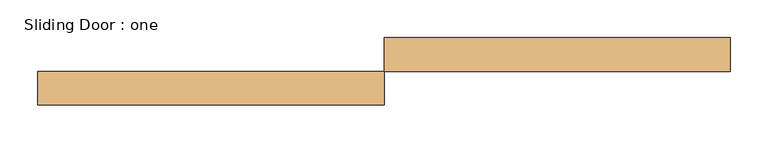
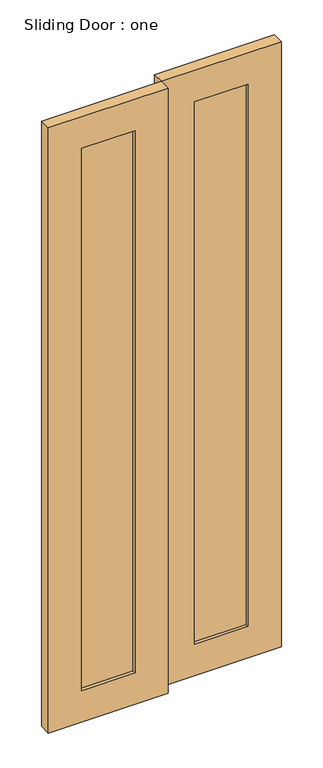
"""IFC4 building model written with IfcOpenShell, lengths in millimetres: door geometry, Sliding Door : one."""

import ifcopenshell
import ifcopenshell.guid

model = None  # the IFC model being written
_history = None  # IfcOwnerHistory: only IFC2X3 demands one
_inside = {}  # id of a spatial element -> (the spatial element, [elements in it])
_under = {}  # id of a project, library or spatial element -> (it, [spatial elements below it])
_declared = {}  # id of a project -> (the project, [libraries it declares])
_typed = {}  # id of a type object -> (the type object, [elements of that type])
_made_of = {}  # id of a material, layer set ... -> (it, [elements and type objects made of it])


def new_model(schema):
    """Start an empty IFC model of exactly this schema.

    Asked for "IFC4X3", IfcOpenShell would pick the latest addendum, in which some entities
    have other attributes; the version numbers below select the first issue.
    IFC2X3 requires an IfcOwnerHistory on every rooted entity: one is made here for all.
    """
    global model, _history
    if schema == "IFC4X3":
        model = ifcopenshell.file(schema_version=(4, 3, 0, 0))
    else:
        model = ifcopenshell.file(schema=schema)
    _inside.clear()
    _under.clear()
    _declared.clear()
    _typed.clear()
    _made_of.clear()
    _history = None
    if model.schema == "IFC2X3":
        org = make("IfcOrganization", Name="unknown")
        user = make(
            "IfcPersonAndOrganization",
            ThePerson=make("IfcPerson", FamilyName="unknown"),
            TheOrganization=org,
        )
        app = make(
            "IfcApplication",
            ApplicationDeveloper=org,
            Version="unknown",
            ApplicationFullName="unknown",
            ApplicationIdentifier="unknown",
        )
        _history = make(
            "IfcOwnerHistory",
            OwningUser=user,
            OwningApplication=app,
            ChangeAction="ADDED",
            CreationDate=0,
        )
    return model


def make(cls, **values):
    """One entity of the class cls with the attributes given. An attribute that is None is left unset."""
    return model.create_entity(
        cls, **{name: value for name, value in values.items() if value is not None}
    )


def rooted(cls, **values):
    """An entity with a GlobalId (a new one), such as an element, a storey or a relation."""
    return make(cls, GlobalId=ifcopenshell.guid.new(), OwnerHistory=_history, **values)


def si_unit(unit_type, name, prefix=None):
    """IfcSIUnit, for example si_unit("LENGTHUNIT", "METRE", prefix="MILLI")."""
    return make("IfcSIUnit", UnitType=unit_type, Prefix=prefix, Name=name)


def assignment(units):
    """IfcUnitAssignment: the units of a project."""
    return None if units is None else make("IfcUnitAssignment", Units=units)


def point(xyz):
    """IfcCartesianPoint."""
    return None if xyz is None else make("IfcCartesianPoint", Coordinates=xyz)


def direction(xyz):
    """IfcDirection."""
    return None if xyz is None else make("IfcDirection", DirectionRatios=xyz)


def frame(location, z_axis=None, x_axis=None):
    """IfcAxis2Placement3D, a coordinate frame: its origin and axes. An axis left out is left unset."""
    return make(
        "IfcAxis2Placement3D",
        Location=point(location),
        Axis=direction(z_axis),
        RefDirection=direction(x_axis),
    )


def origin():
    """The frame at (0, 0, 0) with its axes left unset."""
    return frame((0.0, 0.0, 0.0))


def place(relative_to, where):
    """IfcLocalPlacement: puts the frame where relative to a parent placement (None: the world)."""
    return make(
        "IfcLocalPlacement", PlacementRelTo=relative_to, RelativePlacement=where
    )


def context(
    kind, dimensions, precision=None, world=None, true_north=None, identifier=None
):
    """IfcGeometricRepresentationContext, for example the 3D "Model" context."""
    return make(
        "IfcGeometricRepresentationContext",
        ContextIdentifier=identifier,
        ContextType=kind,
        CoordinateSpaceDimension=dimensions,
        Precision=precision,
        WorldCoordinateSystem=world,
        TrueNorth=true_north,
    )


def project(units=None, contexts=None):
    """IfcProject with its units and contexts."""
    return rooted(
        "IfcProject",
        Name="project",
        RepresentationContexts=contexts,
        UnitsInContext=assignment(units),
    )


def spatial(cls, under=None, at=None, **own):
    """A site, building, storey or space (cls), placed at a placement, below another one or the project."""
    s = rooted(cls, ObjectPlacement=at, **own)
    if under is not None:
        _under.setdefault(under.id(), (under, []))[1].append(s)
    return s


def polyline(points):
    """IfcPolyline through the points."""
    return make("IfcPolyline", Points=[point(p) for p in points])


def outline(outer, holes=None, kind="AREA"):
    """IfcArbitraryClosedProfileDef: a profile drawn as a closed curve; with holes, ...WithVoids."""
    if holes is None:
        return make("IfcArbitraryClosedProfileDef", ProfileType=kind, OuterCurve=outer)
    return make(
        "IfcArbitraryProfileDefWithVoids",
        ProfileType=kind,
        OuterCurve=outer,
        InnerCurves=holes,
    )


def extrude(swept, where, along, depth):
    """IfcExtrudedAreaSolid: the profile swept, set in the frame where, extruded along a direction by depth."""
    return make(
        "IfcExtrudedAreaSolid",
        SweptArea=swept,
        Position=where,
        ExtrudedDirection=direction(along),
        Depth=depth,
    )


def shape(context_of_items, identifier, shape_type, items):
    """IfcShapeRepresentation: the items that make up one representation, for example the "Body"."""
    return make(
        "IfcShapeRepresentation",
        ContextOfItems=context_of_items,
        RepresentationIdentifier=identifier,
        RepresentationType=shape_type,
        Items=items,
    )


def source(mapping_origin, context_of_items, identifier, shape_type, items):
    """IfcRepresentationMap: a shape defined once, which mapped items show again and again."""
    return make(
        "IfcRepresentationMap",
        MappingOrigin=mapping_origin,
        MappedRepresentation=shape(context_of_items, identifier, shape_type, items),
    )


def transform(
    local_origin,
    x_axis=None,
    y_axis=None,
    z_axis=None,
    scale=None,
    scale2=None,
    scale3=None,
    uniform=True,
):
    """IfcCartesianTransformationOperator3D, or its non-uniform kind. x_axis, y_axis, z_axis: its Axis1, 2, 3."""
    if uniform:
        return make(
            "IfcCartesianTransformationOperator3D",
            Axis1=direction(x_axis),
            Axis2=direction(y_axis),
            LocalOrigin=point(local_origin),
            Scale=scale,
            Axis3=direction(z_axis),
        )
    return make(
        "IfcCartesianTransformationOperator3DnonUniform",
        Axis1=direction(x_axis),
        Axis2=direction(y_axis),
        LocalOrigin=point(local_origin),
        Scale=scale,
        Axis3=direction(z_axis),
        Scale2=scale2,
        Scale3=scale3,
    )


def mapped(mapping_source, mapping_target):
    """IfcMappedItem: shows the shape of a source again, moved by a transform."""
    return make(
        "IfcMappedItem", MappingSource=mapping_source, MappingTarget=mapping_target
    )


def made_of(thing, what):
    """Note that an element or type object is made of a material, layer set ...; save() writes the relation."""
    if what is not None:
        _made_of.setdefault(what.id(), (what, []))[1].append(thing)
    return thing


def element(
    cls,
    number,
    at=None,
    inside=None,
    cuts=None,
    type_object=None,
    material=None,
    context=None,
    identifier="Body",
    shape_type=None,
    held_by="IfcProductDefinitionShape",
    body=None,
    shapes=None,
    **own,
):
    """One element of the class cls, such as IfcWall. Its Tag is "e" and its number.

    at: its placement. inside: the storey or other place that contains it. cuts: it is an
    opening in that element (IfcRelVoidsElement). A single representation is given by context,
    identifier, shape_type and body (its items); several are given by shapes. held_by: the class
    of the entity that holds the representations. save() writes the other relations.
    """
    e = rooted(cls, Tag="e%d" % number, ObjectPlacement=at, **own)
    if body is not None:
        shapes = [shape(context, identifier, shape_type, body)]
    if shapes is not None:
        e.Representation = make(held_by, Representations=shapes)
    if inside is not None:
        _inside.setdefault(inside.id(), (inside, []))[1].append(e)
    if cuts is not None:
        rooted(
            "IfcRelVoidsElement", RelatingBuildingElement=cuts, RelatedOpeningElement=e
        )
    if type_object is not None:
        _typed.setdefault(type_object.id(), (type_object, []))[1].append(e)
    return made_of(e, material)


def aggregate(whole, parts):
    """IfcRelAggregates: a whole, such as a stair, and the parts it consists of."""
    return rooted("IfcRelAggregates", RelatingObject=whole, RelatedObjects=parts)


def save(model, path):
    """Write the relations noted so far, then the file.

    IfcRelAggregates (storeys below a building ...), IfcRelContainedInSpatialStructure (elements
    in a storey), IfcRelDefinesByType, IfcRelAssociatesMaterial and IfcRelDeclares: one each for
    every whole, place, type object, material and project.
    """
    for whole, parts in _under.values():
        aggregate(whole, parts)
    for where, things in _inside.values():
        rooted(
            "IfcRelContainedInSpatialStructure",
            RelatedElements=things,
            RelatingStructure=where,
        )
    for kind, things in _typed.values():
        rooted("IfcRelDefinesByType", RelatedObjects=things, RelatingType=kind)
    for what, things in _made_of.values():
        rooted("IfcRelAssociatesMaterial", RelatedObjects=things, RelatingMaterial=what)
    for by, libraries in _declared.values():
        rooted("IfcRelDeclares", RelatingContext=by, RelatedDefinitions=libraries)
    model.write(path)


def sliding_door_one_cf7842af(model_context):
    return source(origin(), model_context, "Body", "SweptSolid", [
        extrude(outline(polyline([(-127.0, -50.8), (-330.2, -50.8), (-330.2, -31.75), (-127.0, -31.75), (-127.0, -50.8)])), frame((0.0, 0.0, 127.0), z_axis=(0.0, 0.0, 1.0), x_axis=(1.0, 0.0, 0.0)), (0.0, 0.0, 1.0), 2184.4),
        extrude(outline(polyline([(330.2, -6.35), (127.0, -6.35), (127.0, 12.7), (330.2, 12.7), (330.2, -6.35)])), frame((0.0, 0.0, 127.0), z_axis=(0.0, 0.0, 1.0), x_axis=(1.0, 0.0, 0.0)), (0.0, 0.0, 1.0), 2184.4),
        extrude(outline(polyline([(2438.4, -457.2), (0.0, -457.2), (0.0, 0.0), (2438.4, 0.0), (2438.4, -457.2)]), holes=[polyline([(127.0, -127.0), (127.0, -330.2), (2311.4, -330.2), (2311.4, -127.0), (127.0, -127.0)])]), frame((0.0, -63.5, 0.0), z_axis=(0.0, 1.0, 0.0), x_axis=(0.0, 0.0, 1.0)), (0.0, 0.0, 1.0), 44.45),
        extrude(outline(polyline([(2438.4, 0.0), (0.0, 0.0), (0.0, 457.2), (2438.4, 457.2), (2438.4, 0.0)]), holes=[polyline([(127.0, 330.2), (127.0, 127.0), (2311.4, 127.0), (2311.4, 330.2), (127.0, 330.2)])]), frame((0.0, -19.05, 0.0), z_axis=(0.0, 1.0, 0.0), x_axis=(0.0, 0.0, 1.0)), (0.0, 0.0, 1.0), 44.45),
    ])


if __name__ == "__main__":
    model = new_model("IFC4")
    model_context = context("Model", 3, world=origin())
    ifc_project = project(units=[si_unit("LENGTHUNIT", "METRE", prefix="MILLI")], contexts=[model_context])
    site = spatial("IfcSite", under=ifc_project)
    building = spatial("IfcBuilding", under=site)
    placement = place(None, origin())
    sliding_door_one_shape = sliding_door_one_cf7842af(model_context)
    element("IfcDoor", 1, ObjectType="Sliding Door : one", at=placement, inside=building, context=model_context, shape_type="MappedRepresentation", body=[
        mapped(sliding_door_one_shape, transform((0.0, 0.0, 0.0), x_axis=(1.0, 0.0, 0.0), y_axis=(0.0, 1.0, 0.0), z_axis=(0.0, 0.0, 1.0))),
    ])
    save(model, "model.ifc")

# Revit data of these elements
# Type "Sliding Door : one"
#   Type Mark = "42"
#   Analytic Construction = "<None>"
#   Stile_Width = 0' - 5"
#   Door_Thickness = 0' - 1 3/4"
#   Door_Offset = 0' - 1"
#   Glass_Material = SAFETY GLAZING
#   Frame_Material = INTERIOR GRADE ALUMINUM STOREFRONT W/ SAFETY GLAZING
#   Function = (empty or 0)
# Element 1 (IfcDoor, "Sliding Door : one")
#   Materials on its faces: "INTERIOR GRADE ALUMINUM STOREFRONT W/ SAFETY GLAZING", "SAFETY GLAZING"
# Materials
#   "SAFETY GLAZING": class "Glass", colour RGB 142 168 196, transparency 0.75, Description = "Soda Lime Glass", Cost = 0
#   "INTERIOR GRADE ALUMINUM STOREFRONT W/ SAFETY GLAZING": class "Metal", colour RGB 226 226 226, transparency 0, Description = "Aluminum 6061", Cost = 0
